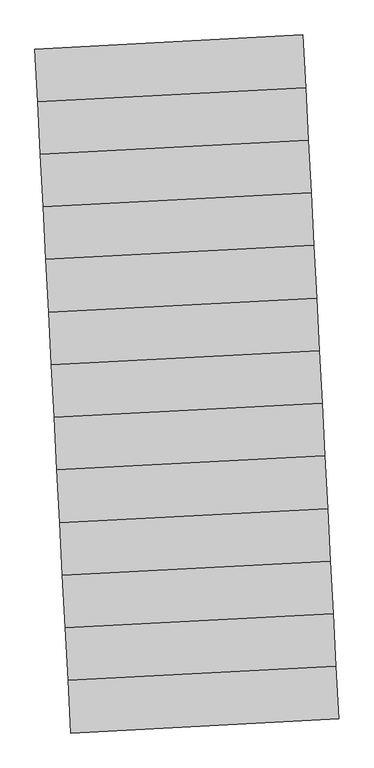
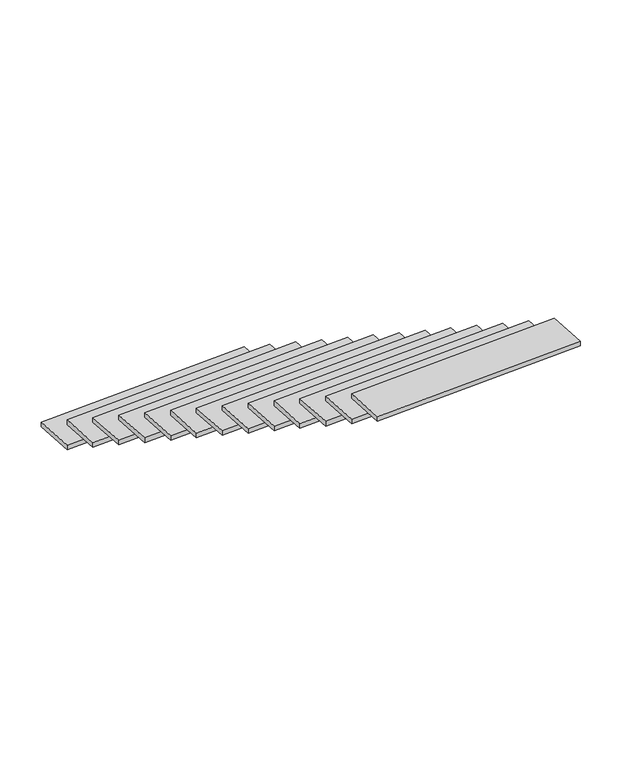
"""IFC4 building model written with IfcOpenShell, lengths in millimetres: stair flight geometry."""

import ifcopenshell
import ifcopenshell.guid

model = None  # the IFC model being written
_history = None  # IfcOwnerHistory: only IFC2X3 demands one
_inside = {}  # id of a spatial element -> (the spatial element, [elements in it])
_under = {}  # id of a project, library or spatial element -> (it, [spatial elements below it])
_declared = {}  # id of a project -> (the project, [libraries it declares])
_typed = {}  # id of a type object -> (the type object, [elements of that type])
_made_of = {}  # id of a material, layer set ... -> (it, [elements and type objects made of it])


def new_model(schema):
    """Start an empty IFC model of exactly this schema.

    Asked for "IFC4X3", IfcOpenShell would pick the latest addendum, in which some entities
    have other attributes; the version numbers below select the first issue.
    IFC2X3 requires an IfcOwnerHistory on every rooted entity: one is made here for all.
    """
    global model, _history
    if schema == "IFC4X3":
        model = ifcopenshell.file(schema_version=(4, 3, 0, 0))
    else:
        model = ifcopenshell.file(schema=schema)
    _inside.clear()
    _under.clear()
    _declared.clear()
    _typed.clear()
    _made_of.clear()
    _history = None
    if model.schema == "IFC2X3":
        org = make("IfcOrganization", Name="unknown")
        user = make(
            "IfcPersonAndOrganization",
            ThePerson=make("IfcPerson", FamilyName="unknown"),
            TheOrganization=org,
        )
        app = make(
            "IfcApplication",
            ApplicationDeveloper=org,
            Version="unknown",
            ApplicationFullName="unknown",
            ApplicationIdentifier="unknown",
        )
        _history = make(
            "IfcOwnerHistory",
            OwningUser=user,
            OwningApplication=app,
            ChangeAction="ADDED",
            CreationDate=0,
        )
    return model


def make(cls, **values):
    """One entity of the class cls with the attributes given. An attribute that is None is left unset."""
    return model.create_entity(
        cls, **{name: value for name, value in values.items() if value is not None}
    )


def rooted(cls, **values):
    """An entity with a GlobalId (a new one), such as an element, a storey or a relation."""
    return make(cls, GlobalId=ifcopenshell.guid.new(), OwnerHistory=_history, **values)


def si_unit(unit_type, name, prefix=None):
    """IfcSIUnit, for example si_unit("LENGTHUNIT", "METRE", prefix="MILLI")."""
    return make("IfcSIUnit", UnitType=unit_type, Prefix=prefix, Name=name)


def assignment(units):
    """IfcUnitAssignment: the units of a project."""
    return None if units is None else make("IfcUnitAssignment", Units=units)


def point(xyz):
    """IfcCartesianPoint."""
    return None if xyz is None else make("IfcCartesianPoint", Coordinates=xyz)


def direction(xyz):
    """IfcDirection."""
    return None if xyz is None else make("IfcDirection", DirectionRatios=xyz)


def frame(location, z_axis=None, x_axis=None):
    """IfcAxis2Placement3D, a coordinate frame: its origin and axes. An axis left out is left unset."""
    return make(
        "IfcAxis2Placement3D",
        Location=point(location),
        Axis=direction(z_axis),
        RefDirection=direction(x_axis),
    )


def origin():
    """The frame at (0, 0, 0) with its axes left unset."""
    return frame((0.0, 0.0, 0.0))


def place(relative_to, where):
    """IfcLocalPlacement: puts the frame where relative to a parent placement (None: the world)."""
    return make(
        "IfcLocalPlacement", PlacementRelTo=relative_to, RelativePlacement=where
    )


def context(
    kind, dimensions, precision=None, world=None, true_north=None, identifier=None
):
    """IfcGeometricRepresentationContext, for example the 3D "Model" context."""
    return make(
        "IfcGeometricRepresentationContext",
        ContextIdentifier=identifier,
        ContextType=kind,
        CoordinateSpaceDimension=dimensions,
        Precision=precision,
        WorldCoordinateSystem=world,
        TrueNorth=true_north,
    )


def project(units=None, contexts=None):
    """IfcProject with its units and contexts."""
    return rooted(
        "IfcProject",
        Name="project",
        RepresentationContexts=contexts,
        UnitsInContext=assignment(units),
    )


def spatial(cls, under=None, at=None, **own):
    """A site, building, storey or space (cls), placed at a placement, below another one or the project."""
    s = rooted(cls, ObjectPlacement=at, **own)
    if under is not None:
        _under.setdefault(under.id(), (under, []))[1].append(s)
    return s


def polyline(points):
    """IfcPolyline through the points."""
    return make("IfcPolyline", Points=[point(p) for p in points])


def outline(outer, holes=None, kind="AREA"):
    """IfcArbitraryClosedProfileDef: a profile drawn as a closed curve; with holes, ...WithVoids."""
    if holes is None:
        return make("IfcArbitraryClosedProfileDef", ProfileType=kind, OuterCurve=outer)
    return make(
        "IfcArbitraryProfileDefWithVoids",
        ProfileType=kind,
        OuterCurve=outer,
        InnerCurves=holes,
    )


def extrude(swept, where, along, depth):
    """IfcExtrudedAreaSolid: the profile swept, set in the frame where, extruded along a direction by depth."""
    return make(
        "IfcExtrudedAreaSolid",
        SweptArea=swept,
        Position=where,
        ExtrudedDirection=direction(along),
        Depth=depth,
    )


def shape(context_of_items, identifier, shape_type, items):
    """IfcShapeRepresentation: the items that make up one representation, for example the "Body"."""
    return make(
        "IfcShapeRepresentation",
        ContextOfItems=context_of_items,
        RepresentationIdentifier=identifier,
        RepresentationType=shape_type,
        Items=items,
    )


def source(mapping_origin, context_of_items, identifier, shape_type, items):
    """IfcRepresentationMap: a shape defined once, which mapped items show again and again."""
    return make(
        "IfcRepresentationMap",
        MappingOrigin=mapping_origin,
        MappedRepresentation=shape(context_of_items, identifier, shape_type, items),
    )


def transform(
    local_origin,
    x_axis=None,
    y_axis=None,
    z_axis=None,
    scale=None,
    scale2=None,
    scale3=None,
    uniform=True,
):
    """IfcCartesianTransformationOperator3D, or its non-uniform kind. x_axis, y_axis, z_axis: its Axis1, 2, 3."""
    if uniform:
        return make(
            "IfcCartesianTransformationOperator3D",
            Axis1=direction(x_axis),
            Axis2=direction(y_axis),
            LocalOrigin=point(local_origin),
            Scale=scale,
            Axis3=direction(z_axis),
        )
    return make(
        "IfcCartesianTransformationOperator3DnonUniform",
        Axis1=direction(x_axis),
        Axis2=direction(y_axis),
        LocalOrigin=point(local_origin),
        Scale=scale,
        Axis3=direction(z_axis),
        Scale2=scale2,
        Scale3=scale3,
    )


def mapped(mapping_source, mapping_target):
    """IfcMappedItem: shows the shape of a source again, moved by a transform."""
    return make(
        "IfcMappedItem", MappingSource=mapping_source, MappingTarget=mapping_target
    )


def made_of(thing, what):
    """Note that an element or type object is made of a material, layer set ...; save() writes the relation."""
    if what is not None:
        _made_of.setdefault(what.id(), (what, []))[1].append(thing)
    return thing


def element(
    cls,
    number,
    at=None,
    inside=None,
    cuts=None,
    type_object=None,
    material=None,
    context=None,
    identifier="Body",
    shape_type=None,
    held_by="IfcProductDefinitionShape",
    body=None,
    shapes=None,
    **own,
):
    """One element of the class cls, such as IfcWall. Its Tag is "e" and its number.

    at: its placement. inside: the storey or other place that contains it. cuts: it is an
    opening in that element (IfcRelVoidsElement). A single representation is given by context,
    identifier, shape_type and body (its items); several are given by shapes. held_by: the class
    of the entity that holds the representations. save() writes the other relations.
    """
    e = rooted(cls, Tag="e%d" % number, ObjectPlacement=at, **own)
    if body is not None:
        shapes = [shape(context, identifier, shape_type, body)]
    if shapes is not None:
        e.Representation = make(held_by, Representations=shapes)
    if inside is not None:
        _inside.setdefault(inside.id(), (inside, []))[1].append(e)
    if cuts is not None:
        rooted(
            "IfcRelVoidsElement", RelatingBuildingElement=cuts, RelatedOpeningElement=e
        )
    if type_object is not None:
        _typed.setdefault(type_object.id(), (type_object, []))[1].append(e)
    return made_of(e, material)


def aggregate(whole, parts):
    """IfcRelAggregates: a whole, such as a stair, and the parts it consists of."""
    return rooted("IfcRelAggregates", RelatingObject=whole, RelatedObjects=parts)


def save(model, path):
    """Write the relations noted so far, then the file.

    IfcRelAggregates (storeys below a building ...), IfcRelContainedInSpatialStructure (elements
    in a storey), IfcRelDefinesByType, IfcRelAssociatesMaterial and IfcRelDeclares: one each for
    every whole, place, type object, material and project.
    """
    for whole, parts in _under.values():
        aggregate(whole, parts)
    for where, things in _inside.values():
        rooted(
            "IfcRelContainedInSpatialStructure",
            RelatedElements=things,
            RelatingStructure=where,
        )
    for kind, things in _typed.values():
        rooted("IfcRelDefinesByType", RelatedObjects=things, RelatingType=kind)
    for what, things in _made_of.values():
        rooted("IfcRelAssociatesMaterial", RelatedObjects=things, RelatingMaterial=what)
    for by, libraries in _declared.values():
        rooted("IfcRelDeclares", RelatingContext=by, RelatedDefinitions=libraries)
    model.write(path)


def stair_flight_a1ef9462(model_context):
    return source(origin(), model_context, "Body", "SweptSolid", [
        extrude(outline(polyline([(25892.6158584, 15125.08554), (24519.5002481, 15053.1236002), (24505.3695399, 15322.7535746), (25878.4851502, 15394.7155144), (25892.6158584, 15125.08554)])), frame((0.0, 0.0, 1768.0), z_axis=(0.0, 0.0, 1.0), x_axis=(1.0, 0.0, 0.0)), (0.0, 0.0, 1.0), 32.0),
        extrude(outline(polyline([(25906.7465666, 14855.4555657), (24533.6309563, 14783.4936258), (24519.5002481, 15053.1236002), (25892.6158584, 15125.08554), (25906.7465666, 14855.4555657)])), frame((0.0, 0.0, 1943.0), z_axis=(0.0, 0.0, 1.0), x_axis=(1.0, 0.0, 0.0)), (0.0, 0.0, 1.0), 32.0),
        extrude(outline(polyline([(25920.8772748, 14585.8255913), (24547.7616645, 14513.8636514), (24533.6309563, 14783.4936258), (25906.7465666, 14855.4555657), (25920.8772748, 14585.8255913)])), frame((0.0, 0.0, 2118.0), z_axis=(0.0, 0.0, 1.0), x_axis=(1.0, 0.0, 0.0)), (0.0, 0.0, 1.0), 32.0),
        extrude(outline(polyline([(25935.007983, 14316.1956169), (24561.8923727, 14244.2336771), (24547.7616645, 14513.8636514), (25920.8772748, 14585.8255913), (25935.007983, 14316.1956169)])), frame((0.0, 0.0, 2293.0), z_axis=(0.0, 0.0, 1.0), x_axis=(1.0, 0.0, 0.0)), (0.0, 0.0, 1.0), 32.0),
        extrude(outline(polyline([(25949.1386911, 14046.5656425), (24576.0230809, 13974.6037027), (24561.8923727, 14244.2336771), (25935.007983, 14316.1956169), (25949.1386911, 14046.5656425)])), frame((0.0, 0.0, 2468.0), z_axis=(0.0, 0.0, 1.0), x_axis=(1.0, 0.0, 0.0)), (0.0, 0.0, 1.0), 32.0),
        extrude(outline(polyline([(25963.2693993, 13776.9356681), (24590.153789, 13704.9737283), (24576.0230809, 13974.6037027), (25949.1386911, 14046.5656425), (25963.2693993, 13776.9356681)])), frame((0.0, 0.0, 2643.0), z_axis=(0.0, 0.0, 1.0), x_axis=(1.0, 0.0, 0.0)), (0.0, 0.0, 1.0), 32.0),
        extrude(outline(polyline([(25977.4001075, 13507.3056937), (24604.2844972, 13435.3437539), (24590.153789, 13704.9737283), (25963.2693993, 13776.9356681), (25977.4001075, 13507.3056937)])), frame((0.0, 0.0, 2818.0), z_axis=(0.0, 0.0, 1.0), x_axis=(1.0, 0.0, 0.0)), (0.0, 0.0, 1.0), 32.0),
        extrude(outline(polyline([(25991.5308157, 13237.6757194), (24618.4152054, 13165.7137795), (24604.2844972, 13435.3437539), (25977.4001075, 13507.3056937), (25991.5308157, 13237.6757194)])), frame((0.0, 0.0, 2993.0), z_axis=(0.0, 0.0, 1.0), x_axis=(1.0, 0.0, 0.0)), (0.0, 0.0, 1.0), 32.0),
        extrude(outline(polyline([(26005.6615239, 12968.045745), (24632.5459136, 12896.0838051), (24618.4152054, 13165.7137795), (25991.5308157, 13237.6757194), (26005.6615239, 12968.045745)])), frame((0.0, 0.0, 3168.0), z_axis=(0.0, 0.0, 1.0), x_axis=(1.0, 0.0, 0.0)), (0.0, 0.0, 1.0), 32.0),
        extrude(outline(polyline([(26019.7922321, 12698.4157706), (24646.6766218, 12626.4538308), (24632.5459136, 12896.0838051), (26005.6615239, 12968.045745), (26019.7922321, 12698.4157706)])), frame((0.0, 0.0, 3343.0), z_axis=(0.0, 0.0, 1.0), x_axis=(1.0, 0.0, 0.0)), (0.0, 0.0, 1.0), 32.0),
        extrude(outline(polyline([(26033.9229403, 12428.7857962), (24660.80733, 12356.8238564), (24646.6766218, 12626.4538308), (26019.7922321, 12698.4157706), (26033.9229403, 12428.7857962)])), frame((0.0, 0.0, 3518.0), z_axis=(0.0, 0.0, 1.0), x_axis=(1.0, 0.0, 0.0)), (0.0, 0.0, 1.0), 32.0),
        extrude(outline(polyline([(26048.0536484, 12159.1558218), (24674.9380382, 12087.193882), (24660.80733, 12356.8238564), (26033.9229403, 12428.7857962), (26048.0536484, 12159.1558218)])), frame((0.0, 0.0, 3693.0), z_axis=(0.0, 0.0, 1.0), x_axis=(1.0, 0.0, 0.0)), (0.0, 0.0, 1.0), 32.0),
        extrude(outline(polyline([(26062.1843566, 11889.5258474), (24689.0687463, 11817.5639076), (24674.9380382, 12087.193882), (26048.0536484, 12159.1558218), (26062.1843566, 11889.5258474)])), frame((0.0, 0.0, 3868.0), z_axis=(0.0, 0.0, 1.0), x_axis=(1.0, 0.0, 0.0)), (0.0, 0.0, 1.0), 32.0),
    ])


if __name__ == "__main__":
    model = new_model("IFC4")
    model_context = context("Model", 3, world=origin())
    ifc_project = project(units=[si_unit("LENGTHUNIT", "METRE", prefix="MILLI")], contexts=[model_context])
    site = spatial("IfcSite", under=ifc_project)
    building = spatial("IfcBuilding", under=site)
    placement = place(None, origin())
    stair_flight_shape = stair_flight_a1ef9462(model_context)
    element("IfcStairFlight", 1, at=placement, inside=building, context=model_context, shape_type="MappedRepresentation", body=[
        mapped(stair_flight_shape, transform((0.0, 0.0, 0.0), x_axis=(1.0, 0.0, 0.0), y_axis=(0.0, 1.0, 0.0), z_axis=(0.0, 0.0, 1.0))),
    ])
    save(model, "model.ifc")

# Revit data of these elements
# Element 1 (IfcStairFlight)
#   Materials on its faces: "철강"
# Materials
#   "철강": class "Generic", colour RGB 143 142 141, transparency 0, Description = "철골+가공조립+세우기", Cost = 0
